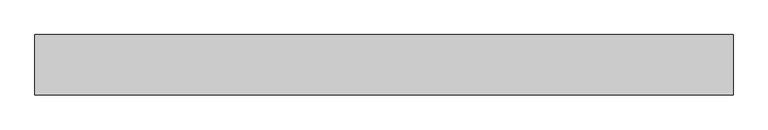
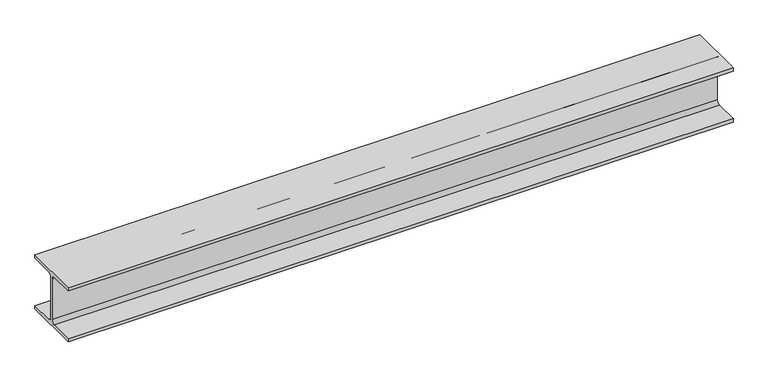
"""IFC4 building model written with IfcOpenShell, lengths in millimetres: beam geometry, 0912_Steel Framing_H-KSD3502 : H_SB_ASB_H-200x200x8x12."""

from ifc_helpers import new_model, si_unit, point, frame, frame_2d, origin, place, context, project, spatial, polyline, circle_curve, trimmed, segment, composite_curve, outline, extrude, source, transform, mapped, element, save


def beam_d4150cb1(model_context):
    return source(origin(), model_context, "Body", "SweptSolid", [
        extrude(outline(composite_curve([segment(polyline([(100.0, -88.0), (100.0, -100.0), (-100.0, -100.0), (-100.0, -88.0), (-17.0, -88.0)]), True, "CONTINUOUS"), segment(trimmed(circle_curve(frame_2d((-17.0, -75.0)), 13.0), [point((-17.0, -88.0))], [point((-4.0, -75.0))], True, "CARTESIAN"), True, "CONTINUOUS"), segment(polyline([(-4.0, -75.0), (-4.0, 75.0)]), True, "CONTINUOUS"), segment(trimmed(circle_curve(frame_2d((-17.0, 75.0)), 13.0), [point((-4.0, 75.0))], [point((-17.0, 88.0))], True, "CARTESIAN"), True, "CONTINUOUS"), segment(polyline([(-17.0, 88.0), (-100.0, 88.0), (-100.0, 100.0), (100.0, 100.0), (100.0, 88.0), (17.0, 88.0)]), True, "CONTINUOUS"), segment(trimmed(circle_curve(frame_2d((17.0, 75.0)), 13.0), [point((17.0, 88.0))], [point((4.0, 75.0))], True, "CARTESIAN"), True, "CONTINUOUS"), segment(polyline([(4.0, 75.0), (4.0, -75.0)]), True, "CONTINUOUS"), segment(trimmed(circle_curve(frame_2d((17.0, -75.0)), 13.0), [point((4.0, -75.0))], [point((17.0, -88.0))], True, "CARTESIAN"), True, "CONTINUOUS"), segment(polyline([(17.0, -88.0), (100.0, -88.0)]), True, "CONTINUOUS")], self_intersect=False)), frame((-1059.9732743, 0.0, 0.0), z_axis=(1.0, 0.0, 0.0), x_axis=(0.0, 1.0, 0.0)), (0.0, 0.0, 1.0), 2315.031312),
    ])


if __name__ == "__main__":
    model = new_model("IFC4")
    model_context = context("Model", 3, world=origin())
    ifc_project = project(units=[si_unit("LENGTHUNIT", "METRE", prefix="MILLI")], contexts=[model_context])
    site = spatial("IfcSite", under=ifc_project)
    building = spatial("IfcBuilding", under=site)
    placement = place(None, origin())
    beam_shape = beam_d4150cb1(model_context)
    element("IfcBeam", 1, ObjectType="0912_Steel Framing_H-KSD3502 : H_SB_ASB_H-200x200x8x12", at=placement, inside=building, context=model_context, shape_type="MappedRepresentation", body=[
        mapped(beam_shape, transform((0.0, 0.0, 0.0), x_axis=(1.0, 0.0, 0.0), y_axis=(0.0, 1.0, 0.0), z_axis=(0.0, 0.0, 1.0))),
    ])
    save(model, "model.ifc")

# Revit data of these elements
# Type "0912_Steel Framing_H-KSD3502 : H_SB_ASB_H-200x200x8x12"
#   H_WM Code_1 = "S01AA002-00001 | Main Steel Structure Fabrication Work | Shelter/Building | Medium Steel - Standard (90KG/M>Weight≥30KG/M) | Material: (   )"
#   H_WM Code_2 = "S03AA028-00001 | Main Steel Structure Erection Work | Shelter/Building | Medium Steel (90KG/M>Weight≥30KG/M) | Material: (   )"
#   H_WM Code_3 = "S01AA010-00001 | Main Steel Structure Fabrication Work | Shelter/Building | Steel Painting/Coating | for Non-Fireproofed Steel Surface, Surface Preparation, Primer, Second & Final Coat | Material: (   )"
#   H_Q'ty Cal Type Tag = "SB-Q2"
#   Width = 20.0 cm
#   Web Thickness = 0.8 cm
#   Web Fillet = 1.3 cm
#   Warping Constant = 141000.0 cm⁶
#   W = 0
#   Torsional Moment of Inertia = 26.2485 cm⁴
#   Section Area = 63.53 cm²
#   Plastic Modulus weak axis = 244.0 cm³
#   Plastic Modulus strong axis = 525.0 cm³
#   Perimeter = 1.16 m²/m
#   Nominal Weight = 49.90 kgf/m
#   Moment of Inertia weak axis = 1600.00 cm⁴
#   Moment of Inertia strong axis = 4720.00 cm⁴
#   Height = 20.0 cm
#   Flange Thickness = 1.2 cm
#   Elastic Modulus weak axis = 160.0 cm³
#   Elastic Modulus strong axis = 472.0 cm³
#   Centroid Vertical = 10.0 cm
#   Centroid Horizontal = 10.0 cm
#   Ix = 47200000
#   Length [instance default] = 1.5240 m
#   Zx = 525000
#   b = 0.2000 m
#   h = 0.2000 m
#   r = 0.0130 m
#   s = 0.0080 m
#   t = 0.0120 m
#   A = 0.006353 m²
#   Structural Material [instance default] = Steel, 45-345
#   Assembly Code = ""
# Element 1 (IfcBeam, "0912_Steel Framing_H-KSD3502 : H_SB_ASB_H-200x200x8x12")
#   Structural Material = none
# Materials
#   "Steel, 45-345": class "Metal", colour RGB 189 187 185, transparency 0, Description = "Steel 345 MPa", Cost = 0
